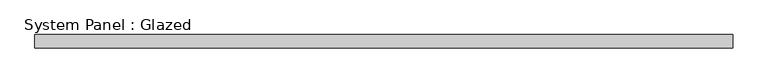
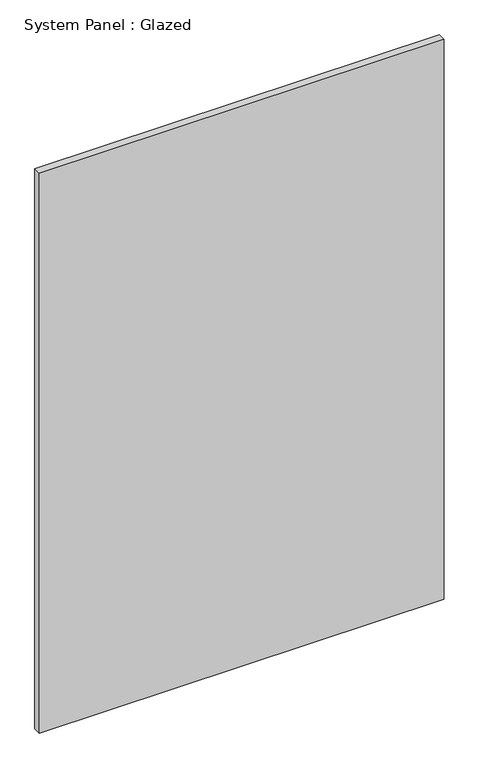
"""IFC4 building model written with IfcOpenShell, lengths in millimetres: plate geometry, System Panel : Glazed."""

from ifc_helpers import new_model, si_unit, origin, origin_with_axes, place, context, project, spatial, polyline, outline, extrude, source, transform, mapped, element, save


def system_panel_glazed_c8739ac2(model_context):
    return source(origin(), model_context, "Body", "SweptSolid", [
        extrude(outline(polyline([(669.7103582, 19.05), (-669.7103582, 19.05), (-669.7103582, 44.45), (669.7103582, 44.45), (669.7103582, 19.05)])), origin_with_axes(), (0.0, 0.0, 1.0), 1957.9166667),
    ])


if __name__ == "__main__":
    model = new_model("IFC4")
    model_context = context("Model", 3, world=origin())
    ifc_project = project(units=[si_unit("LENGTHUNIT", "METRE", prefix="MILLI")], contexts=[model_context])
    site = spatial("IfcSite", under=ifc_project)
    building = spatial("IfcBuilding", under=site)
    placement = place(None, origin())
    system_panel_glazed_shape = system_panel_glazed_c8739ac2(model_context)
    element("IfcPlate", 1, ObjectType="System Panel : Glazed", at=placement, inside=building, context=model_context, shape_type="MappedRepresentation", body=[
        mapped(system_panel_glazed_shape, transform((0.0, 0.0, 0.0), x_axis=(1.0, 0.0, 0.0), y_axis=(0.0, 1.0, 0.0), z_axis=(0.0, 0.0, 1.0))),
    ])
    save(model, "model.ifc")

# Revit data of these elements
# Type "System Panel : Glazed"
#   Construction Type Id = "GSP4R"
#   Analytic Construction = "1/8 in Pilkington single glazing"
#   Visual Light Transmittance = 0.9
#   Solar Heat Gain Coefficient = 0.86
#   Heat Transfer Coefficient (U) = 1.18115 BTU/(h·ft²·°F)
#   Define Thermal Properties by = 1
# Element 1 (IfcPlate, "System Panel : Glazed")
#   Materials on its faces: "Glass"
# Materials
#   "Glass": class "Glass", colour RGB 0 128 192, transparency 0.75, Description = "Soda Lime Glass", Cost = 0
